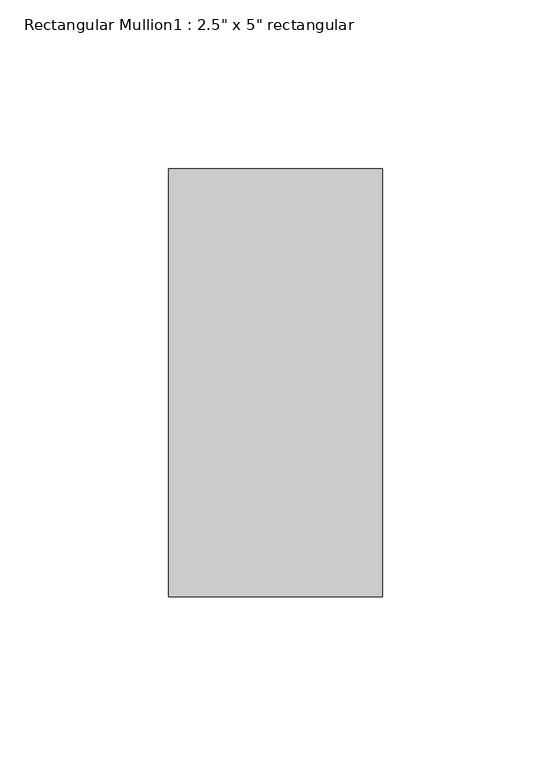
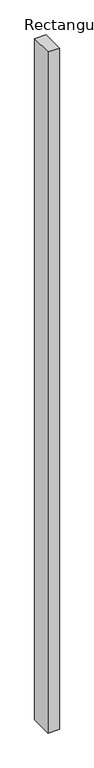
"""IFC4 building model written with IfcOpenShell, lengths in millimetres: member geometry."""

from ifc_helpers import new_model, si_unit, frame, origin, place, context, project, spatial, polyline, outline, extrude, source, transform, mapped, element, save


def member_b283b77b(model_context):
    return source(origin(), model_context, "Body", "SweptSolid", [
        extrude(outline(polyline([(31.75, 63.5), (31.75, -63.5), (-31.75, -63.5), (-31.75, 63.5), (31.75, 63.5)])), frame((0.0, 0.0, -4003.5335741), z_axis=(0.0, 0.0, 1.0), x_axis=(1.0, 0.0, 0.0)), (0.0, 0.0, 1.0), 4003.5335741),
    ])


if __name__ == "__main__":
    model = new_model("IFC4")
    model_context = context("Model", 3, world=origin())
    ifc_project = project(units=[si_unit("LENGTHUNIT", "METRE", prefix="MILLI")], contexts=[model_context])
    site = spatial("IfcSite", under=ifc_project)
    building = spatial("IfcBuilding", under=site)
    placement = place(None, origin())
    member_shape = member_b283b77b(model_context)
    element("IfcMember", 1, ObjectType="Rectangular Mullion1 : 2.5\" x 5\" rectangular", at=placement, inside=building, context=model_context, shape_type="MappedRepresentation", body=[
        mapped(member_shape, transform((0.0, 0.0, 0.0), x_axis=(1.0, 0.0, 0.0), y_axis=(0.0, 1.0, 0.0), z_axis=(0.0, 0.0, 1.0))),
    ])
    save(model, "model.ifc")

# Revit data of these elements
# Type "Rectangular Mullion1 : 2.5\" x 5\" rectangular"
#   built-in parameter 1007304 = 0.416667 (stored number, unit not read)
#   built-in parameter 1007301 = 0.104167 (stored number, unit not read)
#   built-in parameter 1007300 = 0.104167 (stored number, unit not read)
# Element 1 (IfcMember, "Rectangular Mullion1 : 2.5\" x 5\" rectangular")
#   Materials on its faces: "support-frame"
# Materials
#   "support-frame": class "Unassigned", colour RGB 233 233 233, transparency 0, Cost = 0
